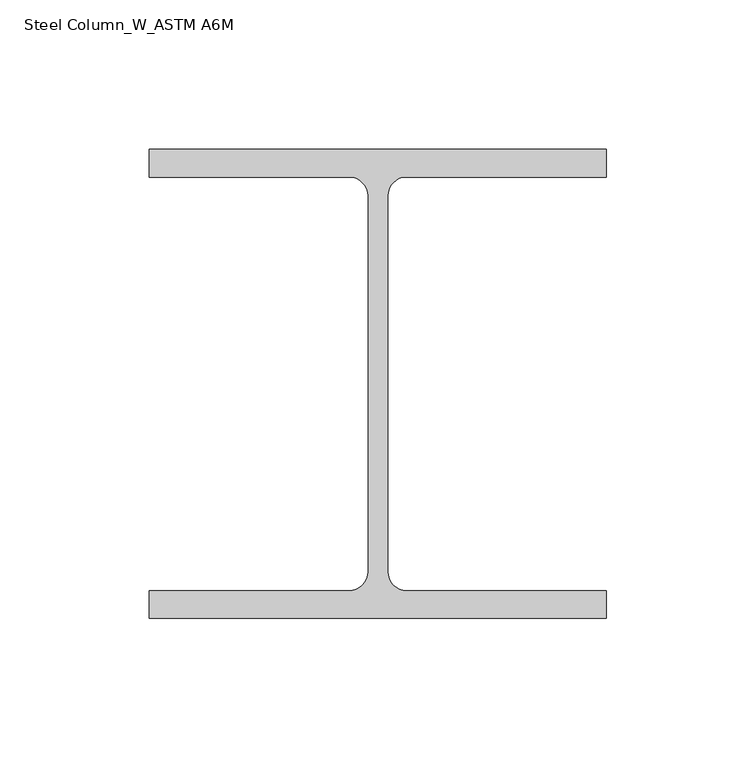
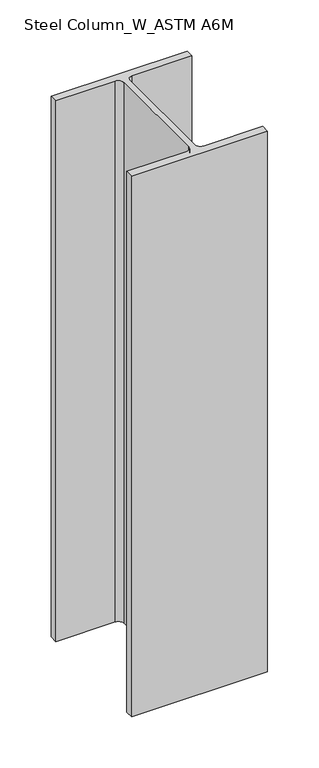
"""IFC4 building model written with IfcOpenShell, lengths in millimetres: column geometry, Steel Column_W_ASTM A6M : H_SC_AR_S01_W150x29.8_P1."""

from ifc_helpers import new_model, si_unit, point, frame, frame_2d, origin, place, context, project, spatial, polyline, circle_curve, trimmed, segment, composite_curve, outline, extrude, source, transform, mapped, element, save


def steel_column_w_astm_a6m_853d7517(model_context):
    return source(origin(), model_context, "Body", "SweptSolid", [
        extrude(outline(composite_curve([segment(polyline([(76.5, 78.5), (76.5, 69.23), (9.63, 69.23)]), True, "CONTINUOUS"), segment(trimmed(circle_curve(frame_2d((9.63, 62.9)), 6.33), [point((9.63, 69.23))], [point((3.3, 62.9))], True, "CARTESIAN"), True, "CONTINUOUS"), segment(polyline([(3.3, 62.9), (3.3, -62.9)]), True, "CONTINUOUS"), segment(trimmed(circle_curve(frame_2d((9.63, -62.9)), 6.33), [point((3.3, -62.9))], [point((9.63, -69.23))], True, "CARTESIAN"), True, "CONTINUOUS"), segment(polyline([(9.63, -69.23), (76.5, -69.23), (76.5, -78.5), (-76.5, -78.5), (-76.5, -69.23), (-9.63, -69.23)]), True, "CONTINUOUS"), segment(trimmed(circle_curve(frame_2d((-9.63, -62.9)), 6.33), [point((-9.63, -69.23))], [point((-3.3, -62.9))], True, "CARTESIAN"), True, "CONTINUOUS"), segment(polyline([(-3.3, -62.9), (-3.3, 62.9)]), True, "CONTINUOUS"), segment(trimmed(circle_curve(frame_2d((-9.63, 62.9)), 6.33), [point((-3.3, 62.9))], [point((-9.63, 69.23))], True, "CARTESIAN"), True, "CONTINUOUS"), segment(polyline([(-9.63, 69.23), (-76.5, 69.23), (-76.5, 78.5), (76.5, 78.5)]), True, "CONTINUOUS")], self_intersect=False)), frame((0.0, 0.0, 1519.8243501), z_axis=(0.0, 0.0, 1.0), x_axis=(1.0, 0.0, 0.0)), (0.0, 0.0, 1.0), 644.0),
    ])


if __name__ == "__main__":
    model = new_model("IFC4")
    model_context = context("Model", 3, world=origin())
    ifc_project = project(units=[si_unit("LENGTHUNIT", "METRE", prefix="MILLI")], contexts=[model_context])
    site = spatial("IfcSite", under=ifc_project)
    building = spatial("IfcBuilding", under=site)
    placement = place(None, origin())
    steel_column_w_astm_a6m_shape = steel_column_w_astm_a6m_853d7517(model_context)
    element("IfcColumn", 1, ObjectType="Steel Column_W_ASTM A6M : H_SC_AR_S01_W150x29.8_P1", at=placement, inside=building, context=model_context, shape_type="MappedRepresentation", body=[
        mapped(steel_column_w_astm_a6m_shape, transform((0.0, 0.0, 0.0), x_axis=(1.0, 0.0, 0.0), y_axis=(0.0, 1.0, 0.0), z_axis=(0.0, 0.0, 1.0))),
    ])
    save(model, "model.ifc")

# Revit data of these elements
# Type "Steel Column_W_ASTM A6M : H_SC_AR_S01_W150x29.8_P1"
#   Section Name Key = "W6x20"
#   Width = 15.3 cm
#   Web Thickness = 0.66 cm
#   Web Fillet = 0.633 cm
#   Warping Constant = 30300.0 cm⁶
#   Torsional Moment of Inertia = 9.99 cm⁴
#   Section Area = 37.9 cm²
#   Plastic Modulus weak axis = 110.0 cm³
#   Plastic Modulus strong axis = 246.0 cm³
#   Perimeter = 0.902 m²/m
#   Nominal Weight = 29.80 kgf/m
#   Moment of Inertia weak axis = 554.00 cm⁴
#   Moment of Inertia strong axis = 1720.00 cm⁴
#   Height = 15.7 cm
#   Flange Thickness = 0.927 cm
#   Elastic Modulus weak axis = 72.3 cm³
#   Elastic Modulus strong axis = 220.0 cm³
#   Centroid Vertical = 7.85 cm
#   Centroid Horizontal = 7.65 cm
#   Structural Material [instance default] = Steel, 45-345
#   Bolt Spacing = 0
#   Assembly Code = ""
# Element 1 (IfcColumn, "Steel Column_W_ASTM A6M : H_SC_AR_S01_W150x29.8_P1")
#   Structural Material = Steel ASTM A992 GRADE 50
#   Materials on its faces: "Steel ASTM A992 GRADE 50"
# Materials
#   "Steel, 45-345": class "Metal", colour RGB 189 187 185, transparency 0, Description = "Steel 345 MPa", Cost = 0
#   "Steel ASTM A992 GRADE 50": class "Metal", colour RGB 120 120 120, transparency 0, Description = "Structural steel 50ksi", Cost = 0
